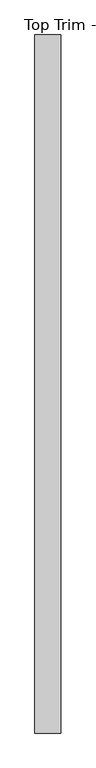
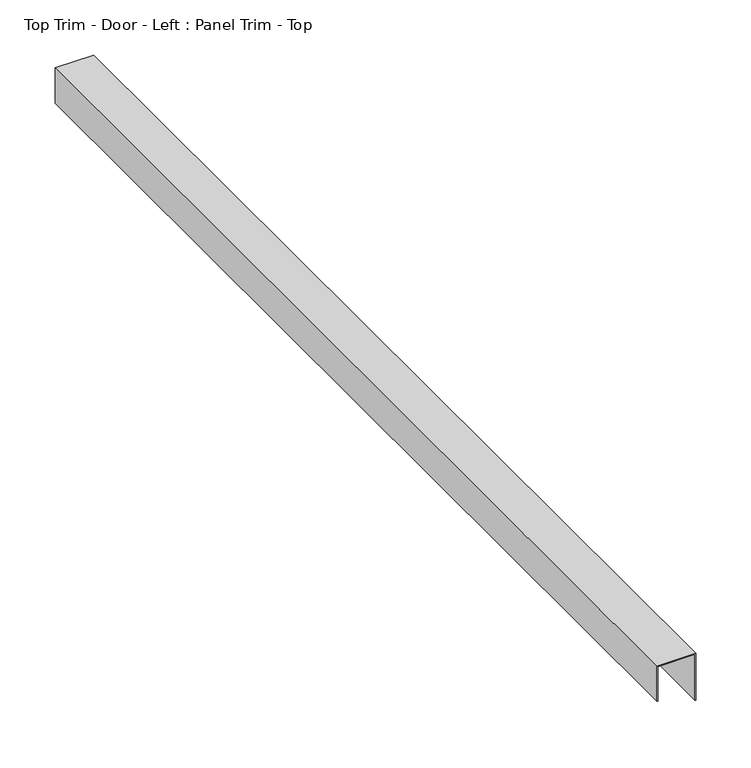
"""IFC4 building model written with IfcOpenShell, lengths in millimetres: proxy geometry, Top Trim - Door - Left : Panel Trim - Top."""

from ifc_helpers import new_model, si_unit, frame, origin, place, context, project, spatial, polyline, outline, extrude, source, transform, mapped, element, save


def top_trim_door_left_panel_trim_top_4d2a0b62(model_context):
    return source(origin(), model_context, "Body", "SweptSolid", [
        extrude(outline(polyline([(2438.4, 587327.0060739), (2438.4, 587365.8934739), (2387.6, 587365.8934739), (2387.6, 587366.6808739), (2439.19375, 587366.6808739), (2439.19375, 587326.2186739), (2400.3, 587326.2186739), (2400.3, 587327.0060739), (2438.4, 587327.0060739)])), frame((0.0, -532877.4663841, 0.0), z_axis=(0.0, 1.0, 0.0), x_axis=(0.0, 0.0, 1.0)), (0.0, 0.0, 1.0), 1092.2),
    ])


if __name__ == "__main__":
    model = new_model("IFC4")
    model_context = context("Model", 3, world=origin())
    ifc_project = project(units=[si_unit("LENGTHUNIT", "METRE", prefix="MILLI")], contexts=[model_context])
    site = spatial("IfcSite", under=ifc_project)
    building = spatial("IfcBuilding", under=site)
    placement = place(None, origin())
    top_trim_door_left_panel_trim_top_shape = top_trim_door_left_panel_trim_top_4d2a0b62(model_context)
    element("IfcBuildingElementProxy", 1, Name="Top Trim - Door - Left : Panel Trim - Top", ObjectType="Top Trim - Door - Left : Panel Trim - Top", at=placement, inside=building, context=model_context, shape_type="MappedRepresentation", body=[
        mapped(top_trim_door_left_panel_trim_top_shape, transform((0.0, 0.0, 0.0), x_axis=(1.0, 0.0, 0.0), y_axis=(0.0, 1.0, 0.0), z_axis=(0.0, 0.0, 1.0))),
    ])
    save(model, "model.ifc")

# Revit data of these elements
# Element 1 (IfcBuildingElementProxy, "Top Trim - Door - Left : Panel Trim - Top")
#   Materials on its faces: "EDGE TRIM BY MTL PANEL MFR."
# Materials
#   "EDGE TRIM BY MTL PANEL MFR.": class "Generic", colour RGB 239 242 240, transparency 0, Cost = 0
